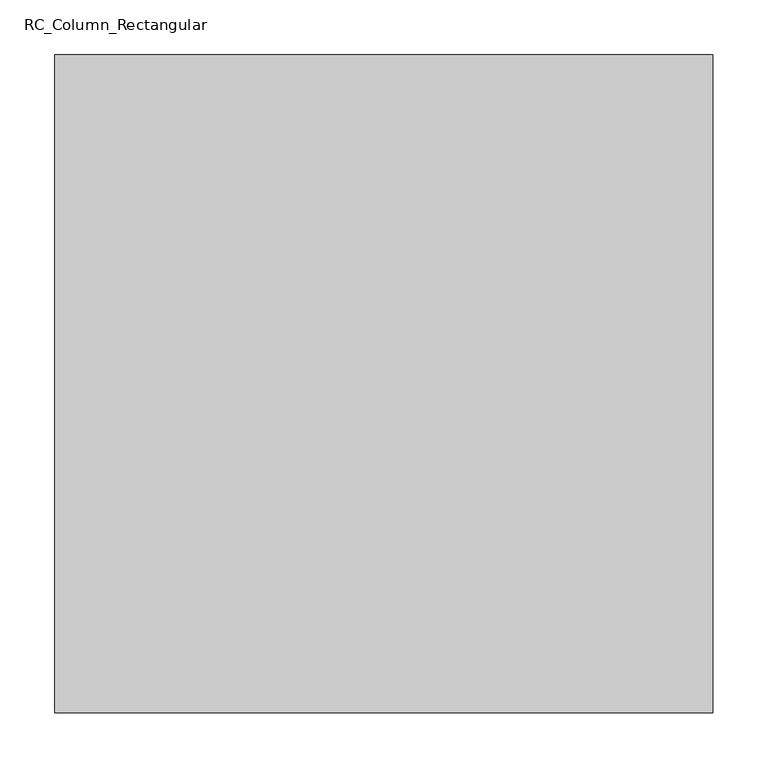
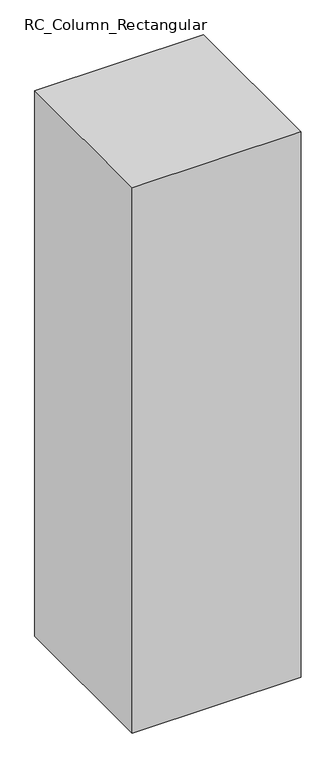
"""IFC4 building model written with IfcOpenShell, lengths in millimetres: column geometry, RC_Column_Rectangular : H_SC_AR_S15_UG PED_W600xL600_Bit_PD2."""

from ifc_helpers import new_model, si_unit, frame, origin, place, context, project, spatial, polyline, outline, extrude, source, transform, mapped, element, save


def rc_column_rectangular_fa199b6f(model_context):
    return source(origin(), model_context, "Body", "SweptSolid", [
        extrude(outline(polyline([(300.0, 300.0), (300.0, -300.0), (-300.0, -300.0), (-300.0, 300.0), (300.0, 300.0)])), frame((0.0, 0.0, -9380.1756499), z_axis=(0.0, 0.0, 1.0), x_axis=(1.0, 0.0, 0.0)), (0.0, 0.0, 1.0), 2050.0),
    ])


if __name__ == "__main__":
    model = new_model("IFC4")
    model_context = context("Model", 3, world=origin())
    ifc_project = project(units=[si_unit("LENGTHUNIT", "METRE", prefix="MILLI")], contexts=[model_context])
    site = spatial("IfcSite", under=ifc_project)
    building = spatial("IfcBuilding", under=site)
    placement = place(None, origin())
    rc_column_rectangular_shape = rc_column_rectangular_fa199b6f(model_context)
    element("IfcColumn", 1, ObjectType="RC_Column_Rectangular : H_SC_AR_S15_UG PED_W600xL600_Bit_PD2", at=placement, inside=building, context=model_context, shape_type="MappedRepresentation", body=[
        mapped(rc_column_rectangular_shape, transform((0.0, 0.0, 0.0), x_axis=(1.0, 0.0, 0.0), y_axis=(0.0, 1.0, 0.0), z_axis=(0.0, 0.0, 1.0))),
    ])
    save(model, "model.ifc")

# Revit data of these elements
# Type "RC_Column_Rectangular : H_SC_AR_S15_UG PED_W600xL600_Bit_PD2"
#   Type Mark = "PD2"
#   Width = 600 mm
#   Length = 600 mm
#   hec_material3 [instance default] = none
#   hec_material2 [instance default] = none
#   hec_material1 [instance default] = none
#   Structural Material [instance default] = none
#   Description = (empty or 0)
